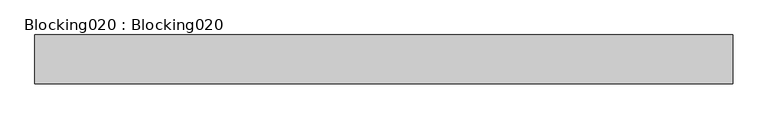
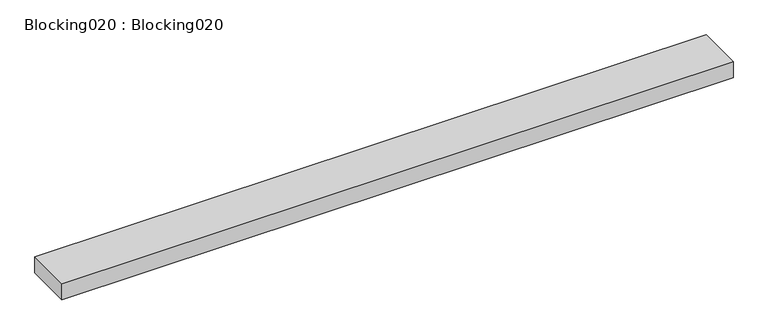
"""IFC4 building model written with IfcOpenShell, lengths in millimetres: proxy geometry, Blocking020 : Blocking020."""

from ifc_helpers import new_model, si_unit, frame, origin, place, context, project, spatial, polyline, outline, extrude, source, transform, mapped, element, save


def blocking020_blocking020_5bf764d7(model_context):
    return source(origin(), model_context, "Body", "SweptSolid", [
        extrude(outline(polyline([(14383.0178845, -4250.1925368), (14383.0178845, -4389.8925368), (12383.0178845, -4389.8925368), (12383.0178845, -4250.1925368), (14383.0178845, -4250.1925368)])), frame((0.0, 0.0, 40112.696), z_axis=(0.0, 0.0, 1.0), x_axis=(1.0, 0.0, 0.0)), (0.0, 0.0, 1.0), 50.8),
    ])


if __name__ == "__main__":
    model = new_model("IFC4")
    model_context = context("Model", 3, world=origin())
    ifc_project = project(units=[si_unit("LENGTHUNIT", "METRE", prefix="MILLI")], contexts=[model_context])
    site = spatial("IfcSite", under=ifc_project)
    building = spatial("IfcBuilding", under=site)
    placement = place(None, origin())
    blocking020_blocking020_shape = blocking020_blocking020_5bf764d7(model_context)
    element("IfcBuildingElementProxy", 1, Name="Blocking020 : Blocking020", ObjectType="Blocking020 : Blocking020", at=placement, inside=building, context=model_context, shape_type="MappedRepresentation", body=[
        mapped(blocking020_blocking020_shape, transform((0.0, 0.0, 0.0), x_axis=(1.0, 0.0, 0.0), y_axis=(0.0, 1.0, 0.0), z_axis=(0.0, 0.0, 1.0))),
    ])
    save(model, "model.ifc")

# Revit data of these elements
# Type "Blocking020 : Blocking020"
#   NameOverride = "Blocking020"
# Element 1 (IfcBuildingElementProxy, "Blocking020 : Blocking020")
#   Materials on its faces: "WOOD BLOCKING AS REQUIRED"
# Materials
#   "WOOD BLOCKING AS REQUIRED": class "Unassigned", colour RGB 166 124 85, transparency 0, Cost = 0
